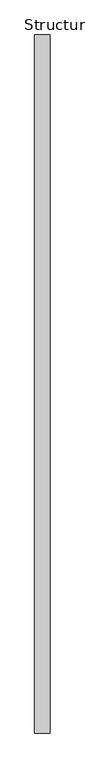
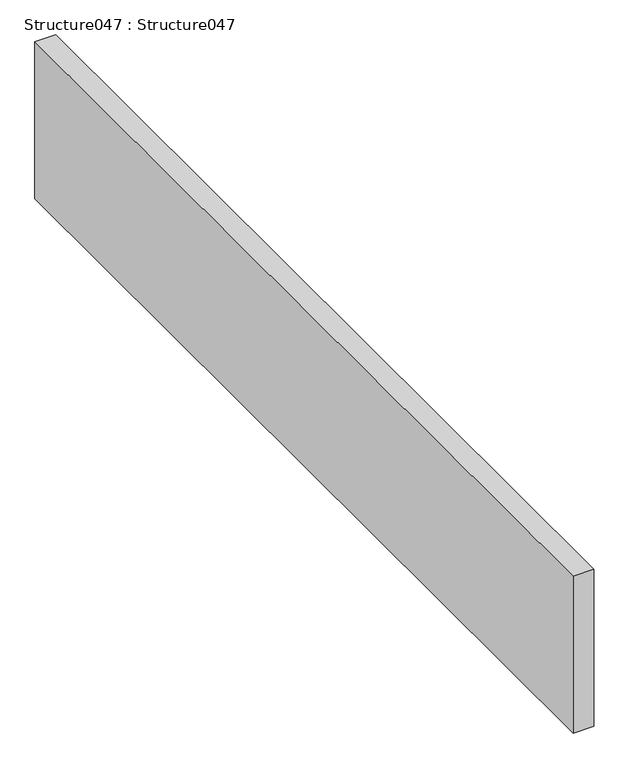
"""IFC4 building model written with IfcOpenShell, lengths in millimetres: proxy geometry, Structure047 : Structure047."""

from ifc_helpers import new_model, si_unit, frame, origin, place, context, project, spatial, polyline, outline, extrude, source, transform, mapped, element, save


def structure047_structure047_5f8ed389(model_context):
    return source(origin(), model_context, "Body", "SweptSolid", [
        extrude(outline(polyline([(-1738.0614422, -1052.8906574), (-1782.5114422, -1052.8906574), (-1782.5114422, 947.1093426), (-1738.0614422, 947.1093426), (-1738.0614422, -1052.8906574)])), frame((0.0, 0.0, 39757.096), z_axis=(0.0, 0.0, 1.0), x_axis=(1.0, 0.0, 0.0)), (0.0, 0.0, 1.0), 355.6),
    ])


if __name__ == "__main__":
    model = new_model("IFC4")
    model_context = context("Model", 3, world=origin())
    ifc_project = project(units=[si_unit("LENGTHUNIT", "METRE", prefix="MILLI")], contexts=[model_context])
    site = spatial("IfcSite", under=ifc_project)
    building = spatial("IfcBuilding", under=site)
    placement = place(None, origin())
    structure047_structure047_shape = structure047_structure047_5f8ed389(model_context)
    element("IfcBuildingElementProxy", 1, Name="Structure047 : Structure047", ObjectType="Structure047 : Structure047", at=placement, inside=building, context=model_context, shape_type="MappedRepresentation", body=[
        mapped(structure047_structure047_shape, transform((0.0, 0.0, 0.0), x_axis=(1.0, 0.0, 0.0), y_axis=(0.0, 1.0, 0.0), z_axis=(0.0, 0.0, 1.0))),
    ])
    save(model, "model.ifc")

# Revit data of these elements
# Type "Structure047 : Structure047"
#   NameOverride = "Structure047"
# Element 1 (IfcBuildingElementProxy, "Structure047 : Structure047")
#   Materials on its faces: "STRUCTURAL MEMBER (SEE DWGS)"
# Materials
#   "STRUCTURAL MEMBER (SEE DWGS)": class "Unassigned", colour RGB 214 178 158, transparency 0, Cost = 0
